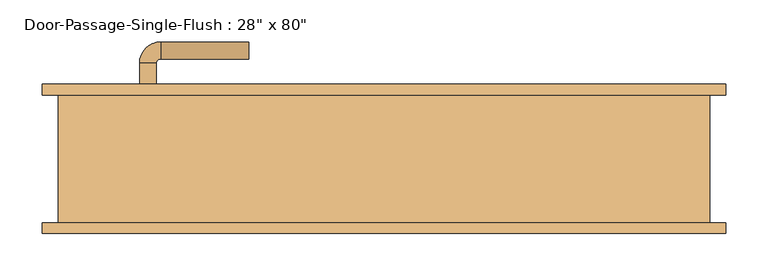
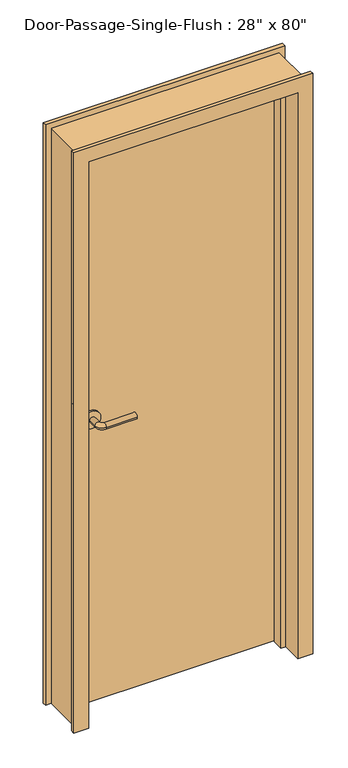
"""IFC4 building model written with IfcOpenShell, lengths in millimetres: door geometry."""

from ifc_helpers import new_model, si_unit, point, frame, frame_2d, origin, origin_with_axes, place, context, project, spatial, polyline, circle_curve, ellipse_curve, trimmed, segment, composite_curve, outline, extrude, faceted_brep, source, transform, mapped, element, save
from ifc_brep_helpers import plane_surface, cylinder_surface, revolved_surface, advanced_brep


def door_4b10be51(model_context):
    return source(origin(), model_context, "Body", "SolidModel", [
        advanced_brep(
        [(-290.590625, 23.75, 1016.0), (-270.590625, 23.75, 1016.0), (-270.590625, -6.25, 1016.0), (-290.590625, -6.25, 1016.0), (-265.590625, -11.25, 1016.0), (-265.590625, -31.25, 1016.0), (-160.590625, -31.25, 1016.0), (-160.590625, -11.25, 1016.0)],
        [
            (0, 1, circle_curve(frame((-280.590625, 23.75, 1016.0), z_axis=(0.0, 1.0, 0.0), x_axis=(1.0, 0.0, 0.0)), 10.0)),
            (1, 0, circle_curve(frame((-280.590625, 23.75, 1016.0), z_axis=(0.0, 1.0, 0.0), x_axis=(1.0, 0.0, 0.0)), 10.0)),
            (1, 2),
            (2, 3, circle_curve(frame((-280.590625, -6.25, 1016.0), z_axis=(0.0, 1.0, 0.0), x_axis=(1.0, 0.0, 0.0)), 10.0)),
            (3, 0),
            (3, 2, circle_curve(frame((-280.590625, -6.25, 1016.0), z_axis=(0.0, 1.0, 0.0), x_axis=(1.0, 0.0, 0.0)), 10.0)),
            (4, 5, circle_curve(frame((-265.590625, -21.25, 1016.0), z_axis=(-1.0, 0.0, 0.0), x_axis=(0.0, 1.0, 0.0)), 10.0)),
            (5, 3, circle_curve(frame((-265.590625, -6.25, 1016.0), z_axis=(0.0, 0.0, -1.0), x_axis=(-1.0, 0.0, 0.0)), 25.0)),
            (2, 4, circle_curve(frame((-265.590625, -6.25, 1016.0), z_axis=(0.0, 0.0, 1.0), x_axis=(-1.0, 0.0, 0.0)), 5.0)),
            (5, 4, circle_curve(frame((-265.590625, -21.25, 1016.0), z_axis=(-1.0, 0.0, 0.0), x_axis=(0.0, 1.0, 0.0)), 10.0)),
            (6, 7, circle_curve(frame((-160.590625, -21.25, 1016.0), z_axis=(1.0, 0.0, 0.0), x_axis=(0.0, 1.0, 0.0)), 10.0)),
            (7, 6, circle_curve(frame((-160.590625, -21.25, 1016.0), z_axis=(1.0, 0.0, 0.0), x_axis=(0.0, 1.0, 0.0)), 10.0)),
            (4, 7),
            (6, 5),
        ],
        [
            plane_surface(frame((-280.590625, 23.75, 1016.0), z_axis=(0.0, 1.0, 0.0), x_axis=(0.0, 0.0, 1.0))),
            cylinder_surface(frame((-280.590625, 23.75, 1016.0), z_axis=(0.0, 1.0, 0.0), x_axis=(1.0, 0.0, 0.0)), 10.0),
            revolved_surface(trimmed(ellipse_curve(frame((-280.590625, -6.25, 1016.0), z_axis=(0.0, -1.0, 0.0), x_axis=(1.0, 0.0, 0.0)), 10.0, 10.0), [point((-290.590625, -6.25, 1016.0))], [point((-270.590625, -6.25, 1016.0))], True, "CARTESIAN"), (-265.590625, -6.25, 1016.0), (0.0, 0.0, -1.0)),
            revolved_surface(trimmed(ellipse_curve(frame((-280.590625, -6.25, 1016.0), z_axis=(0.0, -1.0, 0.0), x_axis=(1.0, 0.0, 0.0)), 10.0, 10.0), [point((-270.590625, -6.25, 1016.0))], [point((-290.590625, -6.25, 1016.0))], True, "CARTESIAN"), (-265.590625, -6.25, 1016.0), (0.0, 0.0, -1.0)),
            plane_surface(frame((-160.590625, -21.25, 1016.0), z_axis=(1.0, 0.0, 0.0), x_axis=(0.0, 0.0, 1.0))),
            cylinder_surface(frame((-265.590625, -21.25, 1016.0), z_axis=(-1.0, 0.0, 0.0), x_axis=(0.0, 1.0, 0.0)), 10.0),
        ],
        [
            (0, [[1, 2]]),
            (1, [[3, 4, 5, -2]]),
            (1, [[-5, 6, -3, -1]]),
            (2, [[7, 8, -4, 9]]),
            (3, [[10, -9, -6, -8]]),
            (4, [[11, 12]]),
            (5, [[13, -11, 14, -7]]),
            (5, [[-14, -12, -13, -10]]),
        ],
    ),
        extrude(outline(composite_curve([segment(trimmed(circle_curve(frame_2d((1016.0, -283.090625)), 30.0), [point((1016.0, -313.090625))], [point((1016.0, -253.090625))], False, "CARTESIAN"), True, "CONTINUOUS"), segment(trimmed(circle_curve(frame_2d((1016.0, -283.090625)), 30.0), [point((1016.0, -253.090625))], [point((1016.0, -313.090625))], False, "CARTESIAN"), True, "CONTINUOUS")], self_intersect=False)), frame((0.0, 23.75, 0.0), z_axis=(0.0, 1.0, 0.0), x_axis=(0.0, 0.0, 1.0)), (0.0, 0.0, 1.0), 8.0),
        advanced_brep(
        [(-290.590625, 90.55, 1016.0), (-270.590625, 90.55, 1016.0), (-290.590625, 120.55, 1016.0), (-270.590625, 120.55, 1016.0), (-265.590625, 125.55, 1016.0), (-265.590625, 145.55, 1016.0), (-160.590625, 145.55, 1016.0), (-160.590625, 125.55, 1016.0)],
        [
            (0, 1, circle_curve(frame((-280.590625, 90.55, 1016.0), z_axis=(0.0, -1.0, 0.0), x_axis=(1.0, 0.0, 0.0)), 10.0)),
            (1, 0, circle_curve(frame((-280.590625, 90.55, 1016.0), z_axis=(0.0, -1.0, 0.0), x_axis=(1.0, 0.0, 0.0)), 10.0)),
            (0, 2),
            (2, 3, circle_curve(frame((-280.590625, 120.55, 1016.0), z_axis=(0.0, -1.0, 0.0), x_axis=(1.0, 0.0, 0.0)), 10.0)),
            (3, 1),
            (3, 2, circle_curve(frame((-280.590625, 120.55, 1016.0), z_axis=(0.0, -1.0, 0.0), x_axis=(1.0, 0.0, 0.0)), 10.0)),
            (4, 3, circle_curve(frame((-265.590625, 120.55, 1016.0), z_axis=(0.0, 0.0, 1.0), x_axis=(-1.0, 0.0, 0.0)), 5.0)),
            (2, 5, circle_curve(frame((-265.590625, 120.55, 1016.0), z_axis=(0.0, 0.0, -1.0), x_axis=(-1.0, 0.0, 0.0)), 25.0)),
            (5, 4, circle_curve(frame((-265.590625, 135.55, 1016.0), z_axis=(-1.0, 0.0, 0.0), x_axis=(0.0, -1.0, 0.0)), 10.0)),
            (4, 5, circle_curve(frame((-265.590625, 135.55, 1016.0), z_axis=(-1.0, 0.0, 0.0), x_axis=(0.0, -1.0, 0.0)), 10.0)),
            (6, 7, circle_curve(frame((-160.590625, 135.55, 1016.0), z_axis=(1.0, 0.0, 0.0), x_axis=(0.0, -1.0, 0.0)), 10.0)),
            (7, 6, circle_curve(frame((-160.590625, 135.55, 1016.0), z_axis=(1.0, 0.0, 0.0), x_axis=(0.0, -1.0, 0.0)), 10.0)),
            (5, 6),
            (7, 4),
        ],
        [
            plane_surface(frame((-280.590625, 90.55, 1016.0), z_axis=(0.0, -1.0, 0.0), x_axis=(0.0, 0.0, 1.0))),
            cylinder_surface(frame((-280.590625, 90.55, 1016.0), z_axis=(0.0, -1.0, 0.0), x_axis=(1.0, 0.0, 0.0)), 10.0),
            revolved_surface(trimmed(ellipse_curve(frame((-280.590625, 120.55, 1016.0), z_axis=(0.0, -1.0, 0.0), x_axis=(1.0, 0.0, 0.0)), 10.0, 10.0), [point((-290.590625, 120.55, 1016.0))], [point((-270.590625, 120.55, 1016.0))], True, "CARTESIAN"), (-265.590625, 120.55, 1016.0), (0.0, 0.0, -1.0)),
            revolved_surface(trimmed(ellipse_curve(frame((-280.590625, 120.55, 1016.0), z_axis=(0.0, -1.0, 0.0), x_axis=(1.0, 0.0, 0.0)), 10.0, 10.0), [point((-270.590625, 120.55, 1016.0))], [point((-290.590625, 120.55, 1016.0))], True, "CARTESIAN"), (-265.590625, 120.55, 1016.0), (0.0, 0.0, -1.0)),
            plane_surface(frame((-160.590625, 135.55, 1016.0), z_axis=(1.0, 0.0, 0.0), x_axis=(0.0, 0.0, 1.0))),
            cylinder_surface(frame((-265.590625, 135.55, 1016.0), z_axis=(-1.0, 0.0, 0.0), x_axis=(0.0, -1.0, 0.0)), 10.0),
        ],
        [
            (0, [[1, 2]]),
            (1, [[-1, 3, 4, 5]]),
            (1, [[-2, -5, 6, -3]]),
            (2, [[7, -4, 8, 9]]),
            (3, [[-8, -6, -7, 10]]),
            (4, [[11, 12]]),
            (5, [[-9, 13, -12, 14]]),
            (5, [[-10, -14, -11, -13]]),
        ],
    ),
        extrude(outline(composite_curve([segment(trimmed(circle_curve(frame_2d((1016.0, -283.090625)), 30.0), [point((1016.0, -313.090625))], [point((1016.0, -253.090625))], False, "CARTESIAN"), True, "CONTINUOUS"), segment(trimmed(circle_curve(frame_2d((1016.0, -283.090625)), 30.0), [point((1016.0, -253.090625))], [point((1016.0, -313.090625))], False, "CARTESIAN"), True, "CONTINUOUS")], self_intersect=False)), frame((0.0, 82.55, 0.0), z_axis=(0.0, 1.0, 0.0), x_axis=(0.0, 0.0, 1.0)), (0.0, 0.0, 1.0), 8.0),
        faceted_brep([(355.6, 95.25, 0.0), (406.4, 95.25, 0.0), (406.4, 82.55, 0.0), (387.35, 82.55, 0.0), (387.35, -69.85, 0.0), (406.4, -69.85, 0.0), (406.4, -82.55, 0.0), (355.6, -82.55, 0.0), (355.6, -11.1125, 0.0), (339.725, -11.1125, 0.0), (339.725, 26.9875, 0.0), (355.6, 26.9875, 0.0), (355.6, 95.25, 2032.0), (-355.6, 95.25, 2032.0), (-355.6, 95.25, 0.0), (-406.4, 95.25, 0.0), (-406.4, 95.25, 2082.8), (406.4, 95.25, 2082.8), (406.4, 82.55, 2082.8), (-406.4, 82.55, 2082.8), (-406.4, 82.55, 0.0), (-387.35, 82.55, 0.0), (-387.35, 82.55, 2063.75), (387.35, 82.55, 2063.75), (387.35, -69.85, 2063.75), (-387.35, -69.85, 2063.75), (-387.35, -69.85, 0.0), (-406.4, -69.85, 0.0), (-406.4, -69.85, 2082.8), (406.4, -69.85, 2082.8), (406.4, -82.55, 2082.8), (-406.4, -82.55, 2082.8), (-406.4, -82.55, 0.0), (-355.6, -82.55, 0.0), (-355.6, -82.55, 2032.0), (355.6, -82.55, 2032.0), (355.6, -11.1125, 2032.0), (-355.6, -11.1125, 2032.0), (-355.6, -11.1125, 0.0), (-339.725, -11.1125, 0.0), (-339.725, -11.1125, 2016.125), (339.725, -11.1125, 2016.125), (339.725, 26.9875, 2016.125), (-339.725, 26.9875, 2016.125), (-339.725, 26.9875, 0.0), (-355.6, 26.9875, 0.0), (-355.6, 26.9875, 2032.0), (355.6, 26.9875, 2032.0)], [[[0, 1, 2, 3, 4, 5, 6, 7, 8, 9, 10, 11]], [[1, 0, 12, 13, 14, 15, 16, 17]], [[2, 1, 17, 18]], [[3, 2, 18, 19, 20, 21, 22, 23]], [[4, 3, 23, 24]], [[5, 4, 24, 25, 26, 27, 28, 29]], [[6, 5, 29, 30]], [[7, 6, 30, 31, 32, 33, 34, 35]], [[8, 7, 35, 36]], [[9, 8, 36, 37, 38, 39, 40, 41]], [[10, 9, 41, 42]], [[11, 10, 42, 43, 44, 45, 46, 47]], [[0, 11, 47, 12]], [[18, 17, 16, 19]], [[24, 23, 22, 25]], [[30, 29, 28, 31]], [[36, 35, 34, 37]], [[42, 41, 40, 43]], [[12, 47, 46, 13]], [[14, 45, 44, 39, 38, 33, 32, 27, 26, 21, 20, 15]], [[19, 16, 15, 20]], [[25, 22, 21, 26]], [[31, 28, 27, 32]], [[37, 34, 33, 38]], [[43, 40, 39, 44]], [[13, 46, 45, 14]]]),
        extrude(outline(polyline([(355.6, 31.75), (-355.6, 31.75), (-355.6, 82.55), (355.6, 82.55), (355.6, 31.75)])), origin_with_axes(), (0.0, 0.0, 1.0), 2032.0),
    ])


if __name__ == "__main__":
    model = new_model("IFC4")
    model_context = context("Model", 3, world=origin())
    ifc_project = project(units=[si_unit("LENGTHUNIT", "METRE", prefix="MILLI")], contexts=[model_context])
    site = spatial("IfcSite", under=ifc_project)
    building = spatial("IfcBuilding", under=site)
    placement = place(None, origin())
    door_shape = door_4b10be51(model_context)
    element("IfcDoor", 1, ObjectType="Door-Passage-Single-Flush : 28\" x 80\"", at=placement, inside=building, context=model_context, shape_type="MappedRepresentation", body=[
        mapped(door_shape, transform((0.0, 0.0, 0.0), x_axis=(1.0, 0.0, 0.0), y_axis=(0.0, 1.0, 0.0), z_axis=(0.0, 0.0, 1.0))),
    ])
    save(model, "model.ifc")

# Revit data of these elements
# Type "Door-Passage-Single-Flush : 28\" x 80\""
#   Type Mark = "15"
#   Assembly Code = "C1020"
#   Analytic Construction = "Wooden"
#   Thickness = 0' - 2"
#   Thermal Resistance (R) = 2.5876 (h·ft²·°F)/BTU
#   Swing Angle [instance default] = 90.00°
#   Strike Height = 3' - 4"
#   Rough Width [instance default] = 2' - 8"
#   Rough Height [instance default] = 7' - 0"
#   Masonry Inset [instance default] = 0' - 1"
#   Masonry Frame Depth = 0' - 5 3/4"
#   MF Opening Width [instance default] = 0' - 4"
#   MF Opening Height [instance default] = 0' - 4"
#   Inset Calculate [instance default] = 0' - 4"
#   Heat Transfer Coefficient (U) = 0.3865 BTU/(h·ft²·°F)
#   Height = 6' - 8"
#   Width = 2' - 4"
#   Masonry Frame [instance default] = yes
#   Dry Wall Frame [instance default] = no
#   Panel Material = Wood - Birch
#   Frame Material = Door - Frame
#   Door Handle Material = Aluminum
#   Visual Light Transmittance = 0
#   Solar Heat Gain Coefficient = 0
#   Function = (empty or 0)
#   Wall Closure = (empty or 0)
# Element 1 (IfcDoor, "Door-Passage-Single-Flush : 28\" x 80\"")
#   Rough Width = 2' - 6 1/2"
#   Rough Height = 6' - 9 1/4"
#   MF Opening Width = 0' - 2 1/2"
#   MF Opening Height = 0' - 1 1/4"
#   Inset Calculate = 0' - 3"
#   Masonry Frame = no
#   Dry Wall Frame = yes
#   Materials on its faces: "Door - Frame", "Aluminum", "Wood - Birch"
# Materials
#   "Wood - Birch": class "Unassigned", colour RGB 224 178 126, transparency 0
#   "Door - Frame": class "Unassigned", colour RGB 118 70 51, transparency 0
#   "Aluminum": class "Metal", colour RGB 244 244 244, transparency 0, Description = "Aluminum 6061", Cost = 0
